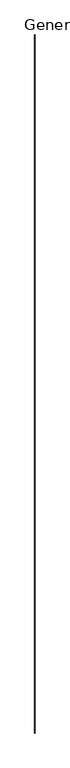
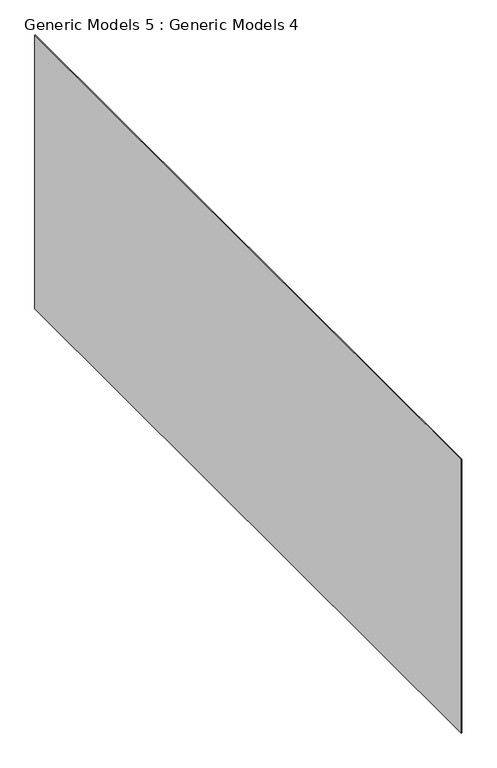
"""IFC4 building model written with IfcOpenShell, lengths in millimetres: proxy geometry, Generic Models 5 : Generic Models 4."""

from ifc_helpers import new_model, si_unit, frame, origin, place, context, project, spatial, polyline, outline, extrude, source, transform, mapped, element, save


def generic_models_5_generic_models_4_6d2c38b6(model_context):
    return source(origin(), model_context, "Body", "SweptSolid", [
        extrude(outline(polyline([(571956.9076893, -527524.3545647), (571956.9076893, -584979.050959), (571931.5076893, -584979.050959), (571931.5076893, -527524.3545647), (571956.9076893, -527524.3545647)])), frame((0.0, 0.0, -2503.337634), z_axis=(0.0, 0.0, 1.0), x_axis=(1.0, 0.0, 0.0)), (0.0, 0.0, 1.0), 22488.6259865),
    ])


if __name__ == "__main__":
    model = new_model("IFC4")
    model_context = context("Model", 3, world=origin())
    ifc_project = project(units=[si_unit("LENGTHUNIT", "METRE", prefix="MILLI")], contexts=[model_context])
    site = spatial("IfcSite", under=ifc_project)
    building = spatial("IfcBuilding", under=site)
    placement = place(None, origin())
    generic_models_5_generic_models_4_shape = generic_models_5_generic_models_4_6d2c38b6(model_context)
    element("IfcBuildingElementProxy", 1, Name="Generic Models 5 : Generic Models 4", ObjectType="Generic Models 5 : Generic Models 4", at=placement, inside=building, context=model_context, shape_type="MappedRepresentation", body=[
        mapped(generic_models_5_generic_models_4_shape, transform((0.0, 0.0, 0.0), x_axis=(1.0, 0.0, 0.0), y_axis=(0.0, 1.0, 0.0), z_axis=(0.0, 0.0, 1.0))),
    ])
    save(model, "model.ifc")

# Revit data of these elements
# Element 1 (IfcBuildingElementProxy, "Generic Models 5 : Generic Models 4")
#   Materials on its faces: "Air"
# Materials
#   "Air": class "Gas", colour RGB 255 255 255, transparency 1, Description = "Air", Cost = 0
